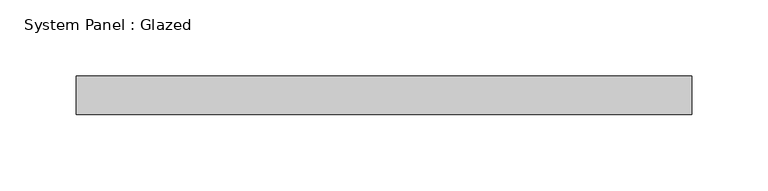
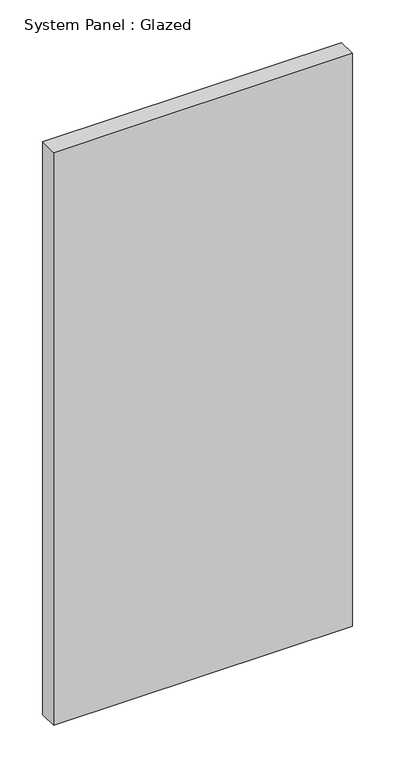
"""IFC4 building model written with IfcOpenShell, lengths in millimetres: plate geometry, System Panel : Glazed."""

from ifc_helpers import new_model, si_unit, origin, origin_with_axes, place, context, project, spatial, polyline, outline, extrude, source, transform, mapped, element, save


def system_panel_glazed_ac6c2aa3(model_context):
    return source(origin(), model_context, "Body", "SweptSolid", [
        extrude(outline(polyline([(202.375, 19.05), (-202.375, 19.05), (-202.375, 44.45), (202.375, 44.45), (202.375, 19.05)])), origin_with_axes(), (0.0, 0.0, 1.0), 819.15),
    ])


if __name__ == "__main__":
    model = new_model("IFC4")
    model_context = context("Model", 3, world=origin())
    ifc_project = project(units=[si_unit("LENGTHUNIT", "METRE", prefix="MILLI")], contexts=[model_context])
    site = spatial("IfcSite", under=ifc_project)
    building = spatial("IfcBuilding", under=site)
    placement = place(None, origin())
    system_panel_glazed_shape = system_panel_glazed_ac6c2aa3(model_context)
    element("IfcPlate", 1, ObjectType="System Panel : Glazed", at=placement, inside=building, context=model_context, shape_type="MappedRepresentation", body=[
        mapped(system_panel_glazed_shape, transform((0.0, 0.0, 0.0), x_axis=(1.0, 0.0, 0.0), y_axis=(0.0, 1.0, 0.0), z_axis=(0.0, 0.0, 1.0))),
    ])
    save(model, "model.ifc")

# Revit data of these elements
# Element 1 (IfcPlate, "System Panel : Glazed")
#   Materials on its faces: "Glass"
# Materials
#   "Glass": class "Glass", colour RGB 0 128 192, transparency 0.75
